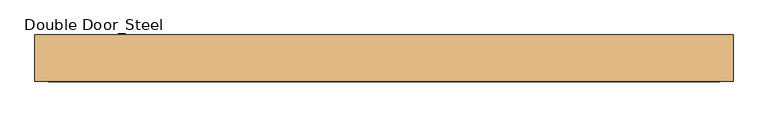
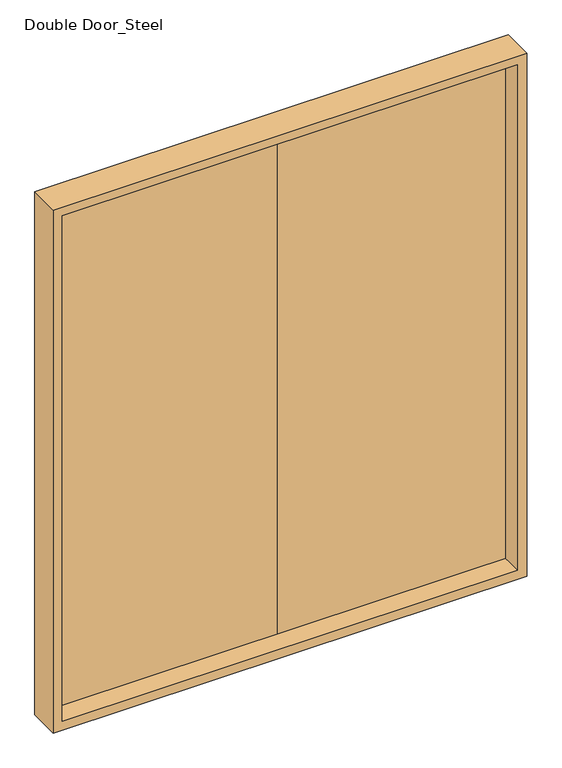
"""IFC4 building model written with IfcOpenShell, lengths in millimetres: door geometry, Double Door_Steel : H_DR_AR_B12_Double Door_Steel_W2000xH2100_0Hr."""

import ifcopenshell
import ifcopenshell.guid

model = None  # the IFC model being written
_history = None  # IfcOwnerHistory: only IFC2X3 demands one
_inside = {}  # id of a spatial element -> (the spatial element, [elements in it])
_under = {}  # id of a project, library or spatial element -> (it, [spatial elements below it])
_declared = {}  # id of a project -> (the project, [libraries it declares])
_typed = {}  # id of a type object -> (the type object, [elements of that type])
_made_of = {}  # id of a material, layer set ... -> (it, [elements and type objects made of it])


def new_model(schema):
    """Start an empty IFC model of exactly this schema.

    Asked for "IFC4X3", IfcOpenShell would pick the latest addendum, in which some entities
    have other attributes; the version numbers below select the first issue.
    IFC2X3 requires an IfcOwnerHistory on every rooted entity: one is made here for all.
    """
    global model, _history
    if schema == "IFC4X3":
        model = ifcopenshell.file(schema_version=(4, 3, 0, 0))
    else:
        model = ifcopenshell.file(schema=schema)
    _inside.clear()
    _under.clear()
    _declared.clear()
    _typed.clear()
    _made_of.clear()
    _history = None
    if model.schema == "IFC2X3":
        org = make("IfcOrganization", Name="unknown")
        user = make(
            "IfcPersonAndOrganization",
            ThePerson=make("IfcPerson", FamilyName="unknown"),
            TheOrganization=org,
        )
        app = make(
            "IfcApplication",
            ApplicationDeveloper=org,
            Version="unknown",
            ApplicationFullName="unknown",
            ApplicationIdentifier="unknown",
        )
        _history = make(
            "IfcOwnerHistory",
            OwningUser=user,
            OwningApplication=app,
            ChangeAction="ADDED",
            CreationDate=0,
        )
    return model


def make(cls, **values):
    """One entity of the class cls with the attributes given. An attribute that is None is left unset."""
    return model.create_entity(
        cls, **{name: value for name, value in values.items() if value is not None}
    )


def rooted(cls, **values):
    """An entity with a GlobalId (a new one), such as an element, a storey or a relation."""
    return make(cls, GlobalId=ifcopenshell.guid.new(), OwnerHistory=_history, **values)


def si_unit(unit_type, name, prefix=None):
    """IfcSIUnit, for example si_unit("LENGTHUNIT", "METRE", prefix="MILLI")."""
    return make("IfcSIUnit", UnitType=unit_type, Prefix=prefix, Name=name)


def assignment(units):
    """IfcUnitAssignment: the units of a project."""
    return None if units is None else make("IfcUnitAssignment", Units=units)


def point(xyz):
    """IfcCartesianPoint."""
    return None if xyz is None else make("IfcCartesianPoint", Coordinates=xyz)


def direction(xyz):
    """IfcDirection."""
    return None if xyz is None else make("IfcDirection", DirectionRatios=xyz)


def frame(location, z_axis=None, x_axis=None):
    """IfcAxis2Placement3D, a coordinate frame: its origin and axes. An axis left out is left unset."""
    return make(
        "IfcAxis2Placement3D",
        Location=point(location),
        Axis=direction(z_axis),
        RefDirection=direction(x_axis),
    )


def origin():
    """The frame at (0, 0, 0) with its axes left unset."""
    return frame((0.0, 0.0, 0.0))


def place(relative_to, where):
    """IfcLocalPlacement: puts the frame where relative to a parent placement (None: the world)."""
    return make(
        "IfcLocalPlacement", PlacementRelTo=relative_to, RelativePlacement=where
    )


def context(
    kind, dimensions, precision=None, world=None, true_north=None, identifier=None
):
    """IfcGeometricRepresentationContext, for example the 3D "Model" context."""
    return make(
        "IfcGeometricRepresentationContext",
        ContextIdentifier=identifier,
        ContextType=kind,
        CoordinateSpaceDimension=dimensions,
        Precision=precision,
        WorldCoordinateSystem=world,
        TrueNorth=true_north,
    )


def project(units=None, contexts=None):
    """IfcProject with its units and contexts."""
    return rooted(
        "IfcProject",
        Name="project",
        RepresentationContexts=contexts,
        UnitsInContext=assignment(units),
    )


def spatial(cls, under=None, at=None, **own):
    """A site, building, storey or space (cls), placed at a placement, below another one or the project."""
    s = rooted(cls, ObjectPlacement=at, **own)
    if under is not None:
        _under.setdefault(under.id(), (under, []))[1].append(s)
    return s


def polyline(points):
    """IfcPolyline through the points."""
    return make("IfcPolyline", Points=[point(p) for p in points])


def outline(outer, holes=None, kind="AREA"):
    """IfcArbitraryClosedProfileDef: a profile drawn as a closed curve; with holes, ...WithVoids."""
    if holes is None:
        return make("IfcArbitraryClosedProfileDef", ProfileType=kind, OuterCurve=outer)
    return make(
        "IfcArbitraryProfileDefWithVoids",
        ProfileType=kind,
        OuterCurve=outer,
        InnerCurves=holes,
    )


def extrude(swept, where, along, depth):
    """IfcExtrudedAreaSolid: the profile swept, set in the frame where, extruded along a direction by depth."""
    return make(
        "IfcExtrudedAreaSolid",
        SweptArea=swept,
        Position=where,
        ExtrudedDirection=direction(along),
        Depth=depth,
    )


def faces_of(points, faces, orient=None, outer=None):
    """IfcFace entities. A face is a list of loops; a loop is a list of indices into points, from 0.

    orient and outer hold one flag for each loop. By default every Orientation is true, the
    first loop of a face is its IfcFaceOuterBound and the others are IfcFaceBound.
    """
    made = []
    for i, loops in enumerate(faces):
        bounds = []
        for j, loop in enumerate(loops):
            is_outer = j == 0 if outer is None else outer[i][j]
            bounds.append(
                make(
                    "IfcFaceOuterBound" if is_outer else "IfcFaceBound",
                    Bound=make("IfcPolyLoop", Polygon=[points[k] for k in loop]),
                    Orientation=True if orient is None else orient[i][j],
                )
            )
        made.append(make("IfcFace", Bounds=bounds))
    return made


def faceted_brep(points, faces, orient=None, outer=None, voids=None):
    """IfcFacetedBrep: a solid bounded by flat faces; with voids (closed shells), ...WithVoids."""
    shared = [point(p) for p in points]
    hull = make("IfcClosedShell", CfsFaces=faces_of(shared, faces, orient, outer))
    if voids is None:
        return make("IfcFacetedBrep", Outer=hull)
    return make(
        "IfcFacetedBrepWithVoids",
        Outer=hull,
        Voids=[
            make(cls, CfsFaces=faces_of(shared, fs, o, b)) for cls, fs, o, b in voids
        ],
    )


def shape(context_of_items, identifier, shape_type, items):
    """IfcShapeRepresentation: the items that make up one representation, for example the "Body"."""
    return make(
        "IfcShapeRepresentation",
        ContextOfItems=context_of_items,
        RepresentationIdentifier=identifier,
        RepresentationType=shape_type,
        Items=items,
    )


def source(mapping_origin, context_of_items, identifier, shape_type, items):
    """IfcRepresentationMap: a shape defined once, which mapped items show again and again."""
    return make(
        "IfcRepresentationMap",
        MappingOrigin=mapping_origin,
        MappedRepresentation=shape(context_of_items, identifier, shape_type, items),
    )


def transform(
    local_origin,
    x_axis=None,
    y_axis=None,
    z_axis=None,
    scale=None,
    scale2=None,
    scale3=None,
    uniform=True,
):
    """IfcCartesianTransformationOperator3D, or its non-uniform kind. x_axis, y_axis, z_axis: its Axis1, 2, 3."""
    if uniform:
        return make(
            "IfcCartesianTransformationOperator3D",
            Axis1=direction(x_axis),
            Axis2=direction(y_axis),
            LocalOrigin=point(local_origin),
            Scale=scale,
            Axis3=direction(z_axis),
        )
    return make(
        "IfcCartesianTransformationOperator3DnonUniform",
        Axis1=direction(x_axis),
        Axis2=direction(y_axis),
        LocalOrigin=point(local_origin),
        Scale=scale,
        Axis3=direction(z_axis),
        Scale2=scale2,
        Scale3=scale3,
    )


def mapped(mapping_source, mapping_target):
    """IfcMappedItem: shows the shape of a source again, moved by a transform."""
    return make(
        "IfcMappedItem", MappingSource=mapping_source, MappingTarget=mapping_target
    )


def made_of(thing, what):
    """Note that an element or type object is made of a material, layer set ...; save() writes the relation."""
    if what is not None:
        _made_of.setdefault(what.id(), (what, []))[1].append(thing)
    return thing


def element(
    cls,
    number,
    at=None,
    inside=None,
    cuts=None,
    type_object=None,
    material=None,
    context=None,
    identifier="Body",
    shape_type=None,
    held_by="IfcProductDefinitionShape",
    body=None,
    shapes=None,
    **own,
):
    """One element of the class cls, such as IfcWall. Its Tag is "e" and its number.

    at: its placement. inside: the storey or other place that contains it. cuts: it is an
    opening in that element (IfcRelVoidsElement). A single representation is given by context,
    identifier, shape_type and body (its items); several are given by shapes. held_by: the class
    of the entity that holds the representations. save() writes the other relations.
    """
    e = rooted(cls, Tag="e%d" % number, ObjectPlacement=at, **own)
    if body is not None:
        shapes = [shape(context, identifier, shape_type, body)]
    if shapes is not None:
        e.Representation = make(held_by, Representations=shapes)
    if inside is not None:
        _inside.setdefault(inside.id(), (inside, []))[1].append(e)
    if cuts is not None:
        rooted(
            "IfcRelVoidsElement", RelatingBuildingElement=cuts, RelatedOpeningElement=e
        )
    if type_object is not None:
        _typed.setdefault(type_object.id(), (type_object, []))[1].append(e)
    return made_of(e, material)


def aggregate(whole, parts):
    """IfcRelAggregates: a whole, such as a stair, and the parts it consists of."""
    return rooted("IfcRelAggregates", RelatingObject=whole, RelatedObjects=parts)


def save(model, path):
    """Write the relations noted so far, then the file.

    IfcRelAggregates (storeys below a building ...), IfcRelContainedInSpatialStructure (elements
    in a storey), IfcRelDefinesByType, IfcRelAssociatesMaterial and IfcRelDeclares: one each for
    every whole, place, type object, material and project.
    """
    for whole, parts in _under.values():
        aggregate(whole, parts)
    for where, things in _inside.values():
        rooted(
            "IfcRelContainedInSpatialStructure",
            RelatedElements=things,
            RelatingStructure=where,
        )
    for kind, things in _typed.values():
        rooted("IfcRelDefinesByType", RelatedObjects=things, RelatingType=kind)
    for what, things in _made_of.values():
        rooted("IfcRelAssociatesMaterial", RelatedObjects=things, RelatingMaterial=what)
    for by, libraries in _declared.values():
        rooted("IfcRelDeclares", RelatingContext=by, RelatedDefinitions=libraries)
    model.write(path)


def double_door_steel_0eef26d0(model_context):
    return source(origin(), model_context, "Body", "SolidModel", [
        extrude(outline(polyline([(880.0, 20.0), (0.0, 20.0), (0.0, 60.0), (880.0, 60.0), (880.0, 20.0)])), frame((0.0, 0.0, 20.0), z_axis=(0.0, 0.0, 1.0), x_axis=(1.0, 0.0, 0.0)), (0.0, 0.0, 1.0), 2060.0),
        extrude(outline(polyline([(0.0, 20.0), (-880.0, 20.0), (-880.0, 60.0), (0.0, 60.0), (0.0, 20.0)])), frame((0.0, 0.0, 20.0), z_axis=(0.0, 0.0, 1.0), x_axis=(1.0, 0.0, 0.0)), (0.0, 0.0, 1.0), 2060.0),
        faceted_brep([(900.0, -60.0, 2100.0), (900.0, 60.0, 2100.0), (-900.0, 60.0, 2100.0), (-900.0, -60.0, 2100.0), (865.0, 20.0, 2065.0), (865.0, -60.0, 2065.0), (-865.0, -60.0, 2065.0), (-865.0, 20.0, 2065.0), (880.0, 60.0, 2080.0), (880.0, 20.0, 2080.0), (-880.0, 20.0, 2080.0), (-880.0, 60.0, 2080.0), (-900.0, 60.0, 0.0), (-900.0, -60.0, 0.0), (-865.0, -60.0, 35.0), (-865.0, 20.0, 35.0), (-880.0, 20.0, 20.0), (-880.0, 60.0, 20.0), (900.0, 60.0, 0.0), (880.0, 60.0, 20.0), (900.0, -60.0, 0.0), (865.0, -60.0, 35.0), (865.0, 20.0, 35.0), (880.0, 20.0, 20.0)], [[[0, 1, 2, 3]], [[4, 5, 6, 7]], [[8, 9, 10, 11]], [[3, 2, 12, 13]], [[7, 6, 14, 15]], [[11, 10, 16, 17]], [[18, 12, 2, 1], [8, 11, 17, 19]], [[13, 12, 18, 20]], [[0, 3, 13, 20], [21, 14, 6, 5]], [[15, 14, 21, 22]], [[23, 16, 10, 9], [4, 7, 15, 22]], [[17, 16, 23, 19]], [[20, 18, 1, 0]], [[22, 21, 5, 4]], [[19, 23, 9, 8]]]),
    ])


if __name__ == "__main__":
    model = new_model("IFC4")
    model_context = context("Model", 3, world=origin())
    ifc_project = project(units=[si_unit("LENGTHUNIT", "METRE", prefix="MILLI")], contexts=[model_context])
    site = spatial("IfcSite", under=ifc_project)
    building = spatial("IfcBuilding", under=site)
    placement = place(None, origin())
    double_door_steel_shape = double_door_steel_0eef26d0(model_context)
    element("IfcDoor", 1, ObjectType="Double Door_Steel : H_DR_AR_B12_Double Door_Steel_W2000xH2100_0Hr", at=placement, inside=building, context=model_context, shape_type="MappedRepresentation", body=[
        mapped(double_door_steel_shape, transform((0.0, 0.0, 0.0), x_axis=(1.0, 0.0, 0.0), y_axis=(0.0, 1.0, 0.0), z_axis=(0.0, 0.0, 1.0))),
    ])
    save(model, "model.ifc")

# Revit data of these elements
# Type "Double Door_Steel : H_DR_AR_B12_Double Door_Steel_W2000xH2100_0Hr"
#   Type Mark = "SD2"
#   프레임 = ""
#   철물 = ""
#   유리/마감 = ""
#   위치/개소 = ""
#   부호 = "1/SD"
#   문번호 = ""
#   문기호 = "SD"
#   Analytic Construction = "<None>"
#   Height = 2100 mm
#   Width = 1800 mm
#   Define Thermal Properties by = 1
#   문 틀 = none
#   문 = none
#   Function = (empty or 0)
#   Assembly Code = ""
#   Wall Closure = (empty or 0)
